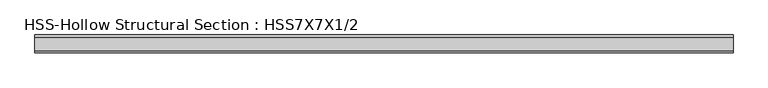
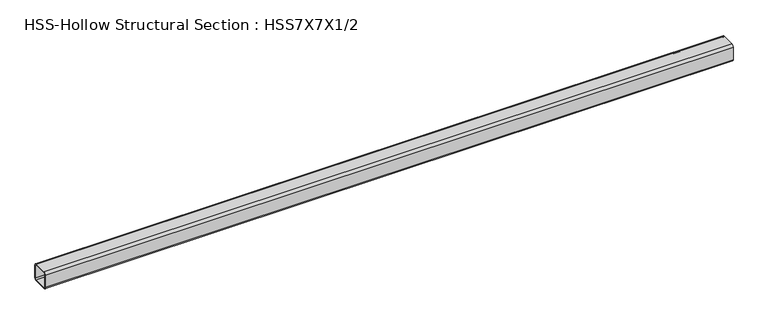
"""IFC4 building model written with IfcOpenShell, lengths in millimetres: member geometry, HSS-Hollow Structural Section : HSS7X7X1/2."""

from ifc_helpers import new_model, si_unit, point, frame, frame_2d, origin, place, context, project, spatial, polyline, circle_curve, trimmed, segment, composite_curve, outline, extrude, source, transform, mapped, element, save


def hss_hollow_structural_section_hss7x7x1_2_33047870(model_context):
    return source(origin(), model_context, "Body", "SweptSolid", [
        extrude(outline(composite_curve([segment(polyline([(88.9, 65.278), (88.9, -65.278)]), True, "CONTINUOUS"), segment(trimmed(circle_curve(frame_2d((65.278, -65.278)), 23.622), [point((88.9, -65.278))], [point((65.278, -88.9))], False, "CARTESIAN"), True, "CONTINUOUS"), segment(polyline([(65.278, -88.9), (-65.278, -88.9)]), True, "CONTINUOUS"), segment(trimmed(circle_curve(frame_2d((-65.278, -65.278)), 23.622), [point((-65.278, -88.9))], [point((-88.9, -65.278))], False, "CARTESIAN"), True, "CONTINUOUS"), segment(polyline([(-88.9, -65.278), (-88.9, 65.278)]), True, "CONTINUOUS"), segment(trimmed(circle_curve(frame_2d((-65.278, 65.278)), 23.622), [point((-88.9, 65.278))], [point((-65.278, 88.9))], False, "CARTESIAN"), True, "CONTINUOUS"), segment(polyline([(-65.278, 88.9), (65.278, 88.9)]), True, "CONTINUOUS"), segment(trimmed(circle_curve(frame_2d((65.278, 65.278)), 23.622), [point((65.278, 88.9))], [point((88.9, 65.278))], False, "CARTESIAN"), True, "CONTINUOUS")], self_intersect=False), holes=[composite_curve([segment(trimmed(circle_curve(frame_2d((-65.278, 65.278)), 11.811), [point((-65.278, 77.089))], [point((-77.089, 65.278))], True, "CARTESIAN"), True, "CONTINUOUS"), segment(polyline([(-77.089, 65.278), (-77.089, -65.278)]), True, "CONTINUOUS"), segment(trimmed(circle_curve(frame_2d((-65.278, -65.278)), 11.811), [point((-77.089, -65.278))], [point((-65.278, -77.089))], True, "CARTESIAN"), True, "CONTINUOUS"), segment(polyline([(-65.278, -77.089), (65.278, -77.089)]), True, "CONTINUOUS"), segment(trimmed(circle_curve(frame_2d((65.278, -65.278)), 11.811), [point((65.278, -77.089))], [point((77.089, -65.278))], True, "CARTESIAN"), True, "CONTINUOUS"), segment(polyline([(77.089, -65.278), (77.089, 65.278)]), True, "CONTINUOUS"), segment(trimmed(circle_curve(frame_2d((65.278, 65.278)), 11.811), [point((77.089, 65.278))], [point((65.278, 77.089))], True, "CARTESIAN"), True, "CONTINUOUS"), segment(polyline([(65.278, 77.089), (-65.278, 77.089)]), True, "CONTINUOUS")], self_intersect=False)]), frame((-3447.6998285, 0.0, 0.0), z_axis=(1.0, 0.0, 0.0), x_axis=(0.0, 1.0, 0.0)), (0.0, 0.0, 1.0), 6895.3996569),
    ])


if __name__ == "__main__":
    model = new_model("IFC4")
    model_context = context("Model", 3, world=origin())
    ifc_project = project(units=[si_unit("LENGTHUNIT", "METRE", prefix="MILLI")], contexts=[model_context])
    site = spatial("IfcSite", under=ifc_project)
    building = spatial("IfcBuilding", under=site)
    placement = place(None, origin())
    hss_hollow_structural_section_hss7x7x1_2_shape = hss_hollow_structural_section_hss7x7x1_2_33047870(model_context)
    element("IfcMember", 1, ObjectType="HSS-Hollow Structural Section : HSS7X7X1/2", at=placement, inside=building, context=model_context, shape_type="MappedRepresentation", body=[
        mapped(hss_hollow_structural_section_hss7x7x1_2_shape, transform((0.0, 0.0, 0.0), x_axis=(1.0, 0.0, 0.0), y_axis=(0.0, 1.0, 0.0), z_axis=(0.0, 0.0, 1.0))),
    ])
    save(model, "model.ifc")

# Revit data of these elements
# Type "HSS-Hollow Structural Section : HSS7X7X1/2"
#   Assembly Code = "B10"
#   Shape = "Square"
#   W = 41.9
#   Ht = 0' - 7"
#   Length [instance default] = 5' - 0"
#   b = 0' - 7"
#   kr = 0' - 0.93"
#   t = 0' - 0.465"
#   A = 0.0805556 SF
#   Structural Material [instance default] = Steel ASTM A500, Grade B, Rectangular and Square
# Element 1 (IfcMember, "HSS-Hollow Structural Section : HSS7X7X1/2")
#   Materials on its faces: "Steel ASTM A500, Grade B, Rectangular and Square"
# Materials
#   "Steel ASTM A500, Grade B, Rectangular and Square": class "Metal", colour RGB 199 199 199, transparency 0, Description = "Carbon steel", Cost = 0
